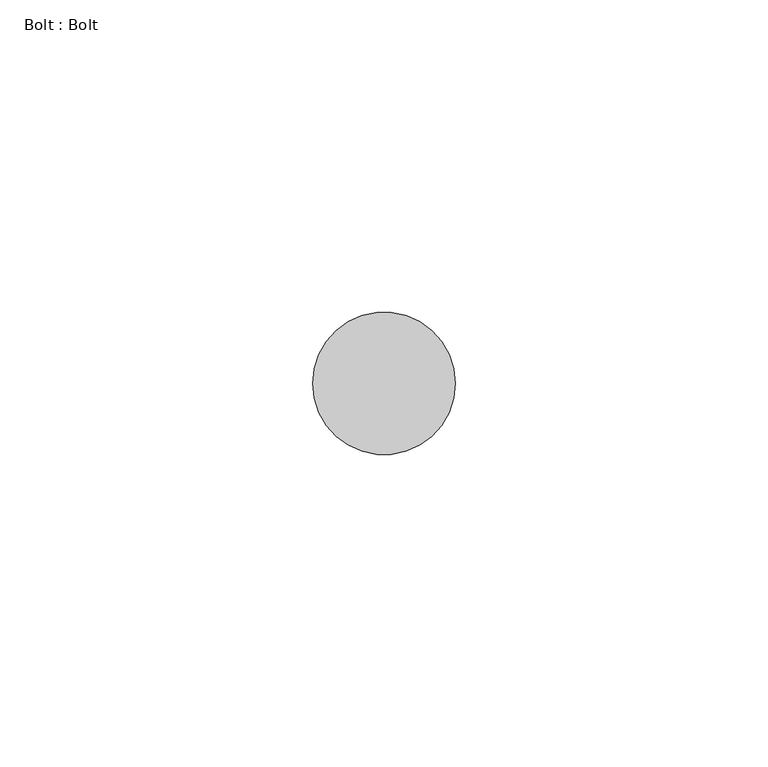
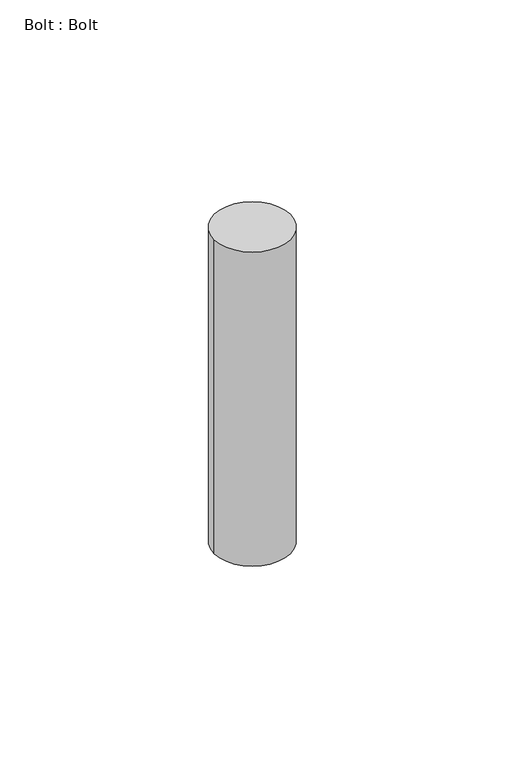
"""IFC4 building model written with IfcOpenShell, lengths in millimetres: proxy geometry, Bolt : Bolt."""

from ifc_helpers import new_model, si_unit, point, frame, frame_2d, origin, place, context, project, spatial, circle_curve, trimmed, segment, composite_curve, outline, extrude, source, transform, mapped, element, save


def bolt_bolt_d23a2250(model_context):
    return source(origin(), model_context, "Body", "SweptSolid", [
        extrude(outline(composite_curve([segment(trimmed(circle_curve(frame_2d((7251.9702148, -1781.8449707)), 11.4045168), [point((7240.565698, -1781.8449707))], [point((7263.3747317, -1781.8449707))], False, "CARTESIAN"), True, "CONTINUOUS"), segment(trimmed(circle_curve(frame_2d((7251.9702148, -1781.8449707)), 11.4045168), [point((7263.3747317, -1781.8449707))], [point((7240.565698, -1781.8449707))], False, "CARTESIAN"), True, "CONTINUOUS")], self_intersect=False)), frame((0.0, 0.0, 39994.0914664), z_axis=(0.0, 0.0, 1.0), x_axis=(1.0, 0.0, 0.0)), (0.0, 0.0, 1.0), 99.5545336),
    ])


if __name__ == "__main__":
    model = new_model("IFC4")
    model_context = context("Model", 3, world=origin())
    ifc_project = project(units=[si_unit("LENGTHUNIT", "METRE", prefix="MILLI")], contexts=[model_context])
    site = spatial("IfcSite", under=ifc_project)
    building = spatial("IfcBuilding", under=site)
    placement = place(None, origin())
    bolt_bolt_shape = bolt_bolt_d23a2250(model_context)
    element("IfcBuildingElementProxy", 1, Name="Bolt : Bolt", ObjectType="Bolt : Bolt", at=placement, inside=building, context=model_context, shape_type="MappedRepresentation", body=[
        mapped(bolt_bolt_shape, transform((0.0, 0.0, 0.0), x_axis=(1.0, 0.0, 0.0), y_axis=(0.0, 1.0, 0.0), z_axis=(0.0, 0.0, 1.0))),
    ])
    save(model, "model.ifc")

# Revit data of these elements
# Type "Bolt : Bolt"
#   NameOverride = "Bolt"
# Element 1 (IfcBuildingElementProxy, "Bolt : Bolt")
#   Materials on its faces: "BOLTS CONCEALED BY FLOOR FINISH"
# Materials
#   "BOLTS CONCEALED BY FLOOR FINISH": class "Unassigned", colour RGB 128 128 128, transparency 0
